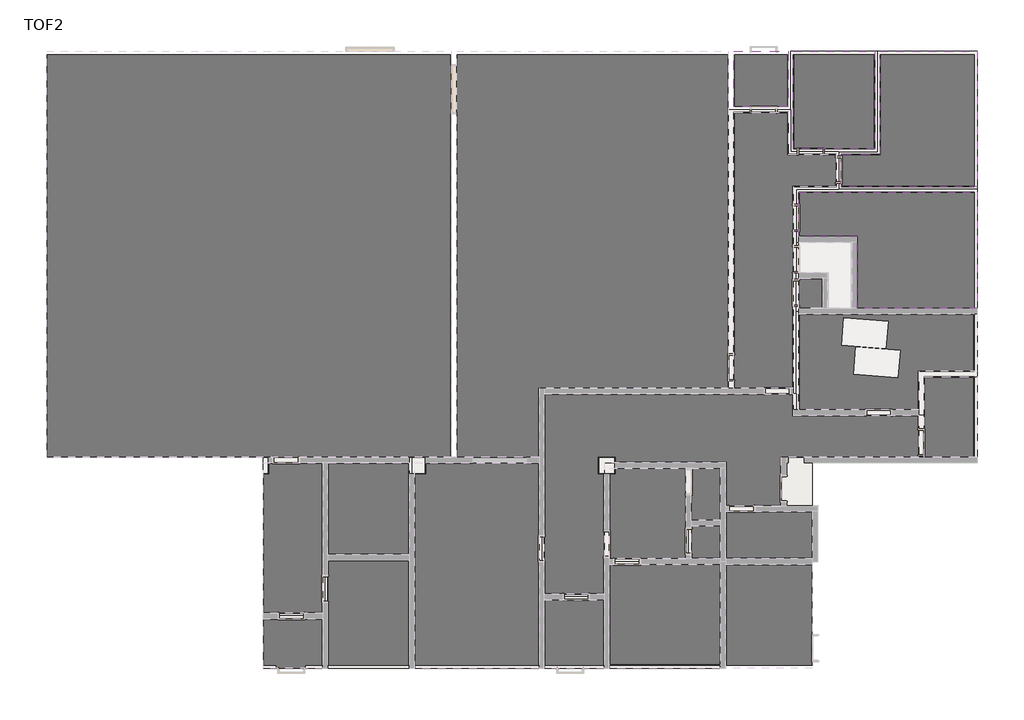
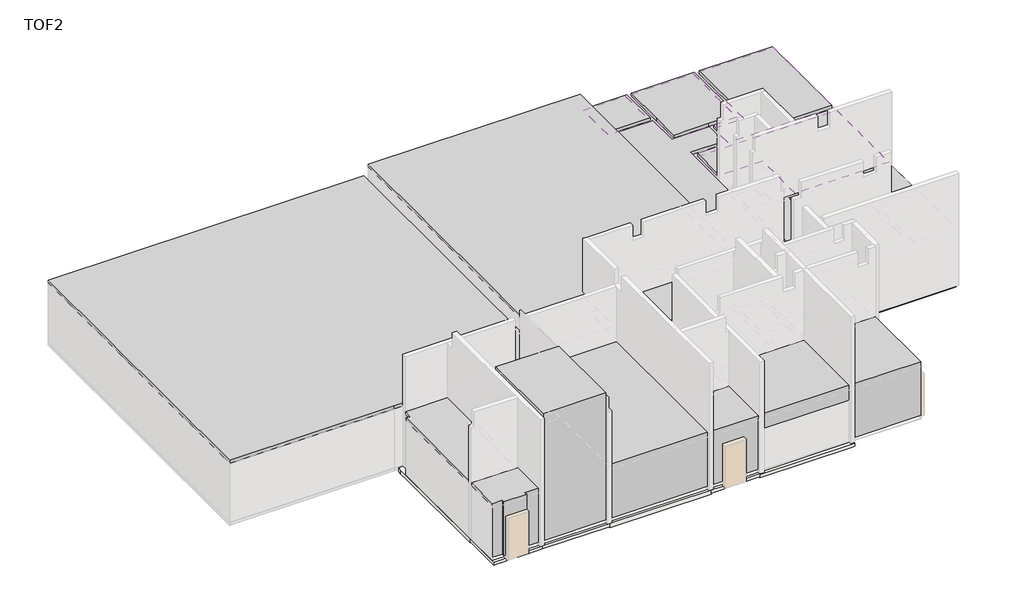
# One storey, part 5 of 5: 24 slabs, 23 proxies, 4 coverings.
# Revit data of these elements (continued)
# Room at (30342.5, 2466.271) mm, phase "New Construction", upper level "TOC", upper offset 2000 mm, lower offset 0 mm (continued)
#   H_Floor Finish-2 = ""
#   H_Floor Finish Remark = ""
#   H_Skirt Base Material = "Same as Wall"
#   H_Skirt-Base Material-1 = ""
#   H_Skirt-Base Material-2 = ""
#   H_Skirt-Base Material-3 = ""
#   H_Skirt-Base Material-4 = ""
#   H_Skirt-Base Material-5 = ""
#   H_Skirt Finish-1 = "Vinyl Tile"
#   H_Skirt Finish-2 = ""
#   H_Skirt Finish Remark = "Vinyl Tile = PVC Tile (polyvinyl chloride)"
#   H_Wall Finish Style Name = "Latex Paint"
#   H_Wall Base Material = "Masonry Wall / Cement Plaster"
#   H_Wall-Base Material-4 = ""
#   H_Wall-Base Material-5 = ""
#   H_Wall Finish-1 = "Latex Paint"
#   H_Wall Finish-2 = ""
#   H_Wall Finish Remark = ""
#   H_Ceiling Finish Style Name = "Acrylic Emulsion Paint"
#   H_Ceiling Base Material = "Concrete Slab / Fair Faced Concrete"
#   H_Ceiling-Base Material-1 = "(Concrete Slab)"
#   H_Ceiling-Base Material-2 = ""
#   H_Ceiling-Base Material-3 = ""
#   H_Ceiling-Base Material-4 = ""
#   H_Ceiling-Base Material-5 = ""
#   H_Ceiling Finish-1 = "Acrylic Emulsion Paint"
#   H_Ceiling Finish-2 = ""
#   H_Ceiling Finish Remark = "SACE"
#   H_Room W = 2900 mm
#   H_Room L = 3300 mm
#   H_Room H or CH = 2600 mm
#   Floor Finish Style No = F34A
#   Skirt Finish Style No = B35
#   Wall Finish Style No = W03B
#   Ceiling Finish Style No = C01
# Room at (30057.5, 6598.271) mm, phase "New Construction", upper level "TOC", upper offset 2000 mm, lower offset 0 mm
#   Comments = ""
#   Number = "113"
#   Name = "STORE"
#   H_Floor Finish Style Name = "Vinyl Tile"
#   H_Floor Base Material = "Concrete Slab / Steel Trowel Finish"
#   H_Wall-Base Material-1 = "Masonry Wall"
#   H_Skirt Finish Style Name = "Coved Vinyl Tile"
#   H_Wall-Base Material-2 = ""
#   H_Wall-Base Material-3 = "Plastering"
#   H_Floor-Base Material-1 = "Concrete Slab"
#   H_Floor-Base Material-2 = "Steel Trowel Finish"
#   H_Floor-Base Material-3 = ""
#   H_Floor-Base Material-4 = ""
#   H_Floor-Base Material-5 = "Vinyl Tile"
#   H_Floor Finish-1 = "Vinyl Tile"
#   H_Floor Finish-2 = ""
#   H_Floor Finish Remark = ""
#   H_Skirt Base Material = "Same as Wall"
#   H_Skirt-Base Material-1 = ""
#   H_Skirt-Base Material-2 = ""
#   H_Skirt-Base Material-3 = ""
#   H_Skirt-Base Material-4 = ""
#   H_Skirt-Base Material-5 = ""
#   H_Skirt Finish-1 = "Vinyl Tile"
#   H_Skirt Finish-2 = ""
#   H_Skirt Finish Remark = "Vinyl Tile = PVC Tile (polyvinyl chloride)"
#   H_Wall Finish Style Name = "Acrylic Emulsion Paint"
#   H_Wall Base Material = "Masonry Wall / Cement Plaster"
#   H_Wall-Base Material-4 = ""
#   H_Wall-Base Material-5 = ""
#   H_Wall Finish-1 = "Acrylic Emulsion Paint"
#   H_Wall Finish-2 = ""
#   H_Wall Finish Remark = "T13 Plaster"
#   H_Ceiling Finish Style Name = "Suspended Acoustic Tiled Ceiling (M-Bar)"
#   H_Ceiling Base Material = "Concrete Slab / Fair Faced Concrete"
#   H_Ceiling-Base Material-1 = "(Concrete Slab)"
#   H_Ceiling-Base Material-2 = "(Fair Faced Concrete)"
#   H_Ceiling-Base Material-3 = ""
#   H_Ceiling-Base Material-4 = ""
#   H_Ceiling-Base Material-5 = "Acoustic Tiled Ceiling System (M-Bar)"
#   H_Ceiling Finish-1 = "Acoustic Tiled Ceiling System (M-Bar)"
#   H_Ceiling Finish-2 = ""
#   H_Ceiling Finish Remark = ""
#   H_Room W = 2100 mm
#   H_Room L = 1900 mm
#   H_Room H or CH = 2700 mm
#   Floor Finish Style No = F34A
#   Skirt Finish Style No = B35
#   Wall Finish Style No = W01B
#   Ceiling Finish Style No = C95A
# Room at (27362.5, 1628.771) mm, phase "New Construction", upper level "TOC", upper offset 2000 mm, lower offset 0 mm
#   Comments = ""
#   Number = "117"
#   Name = "AIR LOCK"
#   H_Floor Finish Style Name = "Vinyl Tile"
#   H_Floor Base Material = "Concrete Slab / Steel Trowel Finish"
#   H_Wall-Base Material-1 = "Masonry Wall"
#   H_Skirt Finish Style Name = "Coved Vinyl Tile"
#   H_Wall-Base Material-2 = ""
#   H_Wall-Base Material-3 = "Plastering"
#   H_Floor-Base Material-1 = "Concrete Slab"
#   H_Floor-Base Material-2 = "Steel Trowel Finish"
#   H_Floor-Base Material-3 = ""
#   H_Floor-Base Material-4 = ""
#   H_Floor-Base Material-5 = "Vinyl Tile"
#   H_Floor Finish-1 = "Vinyl Tile"
#   H_Floor Finish-2 = ""
#   H_Floor Finish Remark = ""
#   H_Skirt Base Material = "Same as Wall"
#   H_Skirt-Base Material-1 = ""
#   H_Skirt-Base Material-2 = ""
#   H_Skirt-Base Material-3 = ""
#   H_Skirt-Base Material-4 = ""
#   H_Skirt-Base Material-5 = ""
#   H_Skirt Finish-1 = "Vinyl Tile"
#   H_Skirt Finish-2 = ""
#   H_Skirt Finish Remark = "Vinyl Tile = PVC Tile (polyvinyl chloride)"
#   H_Wall Finish Style Name = "Acrylic Emulsion Paint"
#   H_Wall Base Material = "Masonry Wall / Cement Plaster"
#   H_Wall-Base Material-4 = ""
#   H_Wall-Base Material-5 = ""
#   H_Wall Finish-1 = "Acrylic Emulsion Paint"
#   H_Wall Finish-2 = ""
#   H_Wall Finish Remark = "T13 Plaster"
#   H_Ceiling Finish Style Name = "Suspended Acoustic Tiled Ceiling (M-Bar)"
#   H_Ceiling Base Material = "Concrete Slab / Fair Faced Concrete"
#   H_Ceiling-Base Material-1 = "(Concrete Slab)"
#   H_Ceiling-Base Material-2 = "(Fair Faced Concrete)"
#   H_Ceiling-Base Material-3 = ""
#   H_Ceiling-Base Material-4 = ""
#   H_Ceiling-Base Material-5 = "Acoustic Tiled Ceiling System (M-Bar)"
#   H_Ceiling Finish-1 = "Acoustic Tiled Ceiling System (M-Bar)"
#   H_Ceiling Finish-2 = ""
#   H_Ceiling Finish Remark = ""
#   H_Room W = 2100 mm
#   H_Room L = 5500 mm
#   H_Room H or CH = 2600 mm
#   Floor Finish Style No = F34A
#   Skirt Finish Style No = B35
#   Wall Finish Style No = W01B
#   Ceiling Finish Style No = C95A
# Room at (27362.5, 5760.771) mm, phase "New Construction", upper level "TOC", upper offset 2000 mm, lower offset 0 mm
#   Comments = ""
#   Number = "116"
#   Name = "CORRIDOR"
#   H_Floor Finish Style Name = "Vinyl Tile"
#   H_Floor Base Material = "Concrete Slab / Steel Trowel Finish"
#   H_Wall-Base Material-1 = "Masonry Wall"
#   H_Skirt Finish Style Name = "Coved Vinyl Tile"
#   H_Wall-Base Material-2 = ""
#   H_Wall-Base Material-3 = "Plastering"
#   H_Floor-Base Material-1 = "Concrete Slab"
#   H_Floor-Base Material-2 = "Steel Trowel Finish"
#   H_Floor-Base Material-3 = ""
#   H_Floor-Base Material-4 = ""
#   H_Floor-Base Material-5 = "Vinyl Tile"
#   H_Floor Finish-1 = "Vinyl Tile"
#   H_Floor Finish-2 = ""
#   H_Floor Finish Remark = ""
#   H_Skirt Base Material = "Same as Wall"
#   H_Skirt-Base Material-1 = ""
#   H_Skirt-Base Material-2 = ""
#   H_Skirt-Base Material-3 = ""
#   H_Skirt-Base Material-4 = ""
#   H_Skirt-Base Material-5 = ""
#   H_Skirt Finish-1 = "Vinyl Tile"
#   H_Skirt Finish-2 = ""
#   H_Skirt Finish Remark = "Vinyl Tile = PVC Tile (polyvinyl chloride)"
#   H_Wall Finish Style Name = "Acrylic Emulsion Paint"
#   H_Wall Base Material = "Masonry Wall / Cement Plaster"
#   H_Wall-Base Material-4 = ""
#   H_Wall-Base Material-5 = ""
#   H_Wall Finish-1 = "Acrylic Emulsion Paint"
#   H_Wall Finish-2 = ""
#   H_Wall Finish Remark = "T13 Plaster"
#   H_Ceiling Finish Style Name = "Suspended Acoustic Tiled Ceiling (M-Bar)"
#   H_Ceiling Base Material = "Concrete Slab / Fair Faced Concrete"
#   H_Ceiling-Base Material-1 = "(Concrete Slab)"
#   H_Ceiling-Base Material-2 = "(Fair Faced Concrete)"
#   H_Ceiling-Base Material-3 = ""
#   H_Ceiling-Base Material-4 = ""
#   H_Ceiling-Base Material-5 = "Acoustic Tiled Ceiling System (M-Bar)"
#   H_Ceiling Finish-1 = "Acoustic Tiled Ceiling System (M-Bar)"
#   H_Ceiling Finish-2 = ""
#   H_Ceiling Finish Remark = ""
#   H_Room W = 13800 mm
#   H_Room L = 7300 mm
#   H_Room H or CH = 2600 mm
#   Floor Finish Style No = F34A
#   Skirt Finish Style No = B35
#   Wall Finish Style No = W01B
#   Ceiling Finish Style No = C95A
# Room at (43870, 7604.869) mm, phase "New Construction", upper level "TOC", upper offset 2000 mm, lower offset 0 mm
#   Comments = ""
#   Number = "120"
#   Name = "CORRIDOR"
#   H_Floor Finish Style Name = "Vinyl Tile"
#   H_Floor Base Material = "Concrete Slab / Steel Trowel Finish"
#   H_Wall-Base Material-1 = "Masonry Wall"
#   H_Skirt Finish Style Name = "Coved Vinyl Tile"
#   H_Wall-Base Material-2 = ""
#   H_Wall-Base Material-3 = "Plastering"
#   H_Floor-Base Material-1 = "Concrete Slab"
#   H_Floor-Base Material-2 = "Steel Trowel Finish"
#   H_Floor-Base Material-3 = ""
#   H_Floor-Base Material-4 = ""
#   H_Floor-Base Material-5 = "Vinyl Tile"
#   H_Floor Finish-1 = "Vinyl Tile"
#   H_Floor Finish-2 = ""
#   H_Floor Finish Remark = ""
#   H_Skirt Base Material = "Same as Wall"
#   H_Skirt-Base Material-1 = ""
#   H_Skirt-Base Material-2 = ""
#   H_Skirt-Base Material-3 = ""
#   H_Skirt-Base Material-4 = ""
#   H_Skirt-Base Material-5 = ""
#   H_Skirt Finish-1 = "Vinyl Tile"
#   H_Skirt Finish-2 = ""
#   H_Skirt Finish Remark = "Vinyl Tile = PVC Tile (polyvinyl chloride)"
#   H_Wall Finish Style Name = "Acrylic Emulsion Paint"
#   H_Wall Base Material = "Masonry Wall / Cement Plaster"
#   H_Wall-Base Material-4 = ""
#   H_Wall-Base Material-5 = ""
#   H_Wall Finish-1 = "Acrylic Emulsion Paint"
#   H_Wall Finish-2 = ""
#   H_Wall Finish Remark = "T13 Plaster"
#   H_Ceiling Finish Style Name = "Suspended Acoustic Tiled Ceiling (M-Bar)"
#   H_Ceiling Base Material = "Concrete Slab / Fair Faced Concrete"
#   H_Ceiling-Base Material-1 = "(Concrete Slab)"
#   H_Ceiling-Base Material-2 = "(Fair Faced Concrete)"
#   H_Ceiling-Base Material-3 = ""
#   H_Ceiling-Base Material-4 = ""
#   H_Ceiling-Base Material-5 = "Acoustic Tiled Ceiling System (M-Bar)"
#   H_Ceiling Finish-1 = "Acoustic Tiled Ceiling System (M-Bar)"
#   H_Ceiling Finish-2 = ""
#   H_Ceiling Finish Remark = ""
#   H_Room W = 2100 mm
#   H_Room L = 2400 mm
#   H_Room H or CH = 2600 mm
#   Floor Finish Style No = F34A
#   Skirt Finish Style No = B35
#   Wall Finish Style No = W01B
#   Ceiling Finish Style No = C95A
# Room at (37870, 1977.173) mm, phase "New Construction", upper level "TOC", upper offset 2000 mm, lower offset 0 mm
#   Comments = ""
#   Number = "119"
#   Name = "AIR LOCK"
#   H_Floor Finish Style Name = "Vinyl Tile"
#   H_Floor Base Material = "Concrete Slab / Steel Trowel Finish"
#   H_Wall-Base Material-1 = "Masonry Wall"
#   H_Skirt Finish Style Name = "Coved Vinyl Tile"
#   H_Wall-Base Material-2 = ""
#   H_Wall-Base Material-3 = "Plastering"
#   H_Floor-Base Material-1 = "Concrete Slab"
#   H_Floor-Base Material-2 = "Steel Trowel Finish"
#   H_Floor-Base Material-3 = ""
#   H_Floor-Base Material-4 = ""
#   H_Floor-Base Material-5 = "Vinyl Tile"
#   H_Floor Finish-1 = "Vinyl Tile"
#   H_Floor Finish-2 = ""
#   H_Floor Finish Remark = ""
#   H_Skirt Base Material = "Same as Wall"
#   H_Skirt-Base Material-1 = ""
#   H_Skirt-Base Material-2 = ""
#   H_Skirt-Base Material-3 = ""
#   H_Skirt-Base Material-4 = ""
#   H_Skirt-Base Material-5 = ""
#   H_Skirt Finish-1 = "Vinyl Tile"
#   H_Skirt Finish-2 = ""
#   H_Skirt Finish Remark = "Vinyl Tile = PVC Tile (polyvinyl chloride)"
#   H_Wall Finish Style Name = "Acrylic Emulsion Paint"
#   H_Wall Base Material = "Masonry Wall / Cement Plaster"
#   H_Wall-Base Material-4 = ""
#   H_Wall-Base Material-5 = ""
#   H_Wall Finish-1 = "Acrylic Emulsion Paint"
#   H_Wall Finish-2 = ""
#   H_Wall Finish Remark = "T13 Plaster"
#   H_Ceiling Finish Style Name = "Suspended Acoustic Tiled Ceiling (M-Bar)"
#   H_Ceiling Base Material = "Concrete Slab / Fair Faced Concrete"
#   H_Ceiling-Base Material-1 = "(Concrete Slab)"
#   H_Ceiling-Base Material-2 = "(Fair Faced Concrete)"
#   H_Ceiling-Base Material-3 = ""
#   H_Ceiling-Base Material-4 = ""
#   H_Ceiling-Base Material-5 = "Acoustic Tiled Ceiling System (M-Bar)"
#   H_Ceiling Finish-1 = "Acoustic Tiled Ceiling System (M-Bar)"
#   H_Ceiling Finish-2 = ""
#   H_Ceiling Finish Remark = ""
#   H_Room W = 2400 mm
#   H_Room L = 2500 mm
#   H_Room H or CH = 2700 mm
#   Floor Finish Style No = F34A
#   Skirt Finish Style No = B35
#   Wall Finish Style No = W01B
#   Ceiling Finish Style No = C95A
